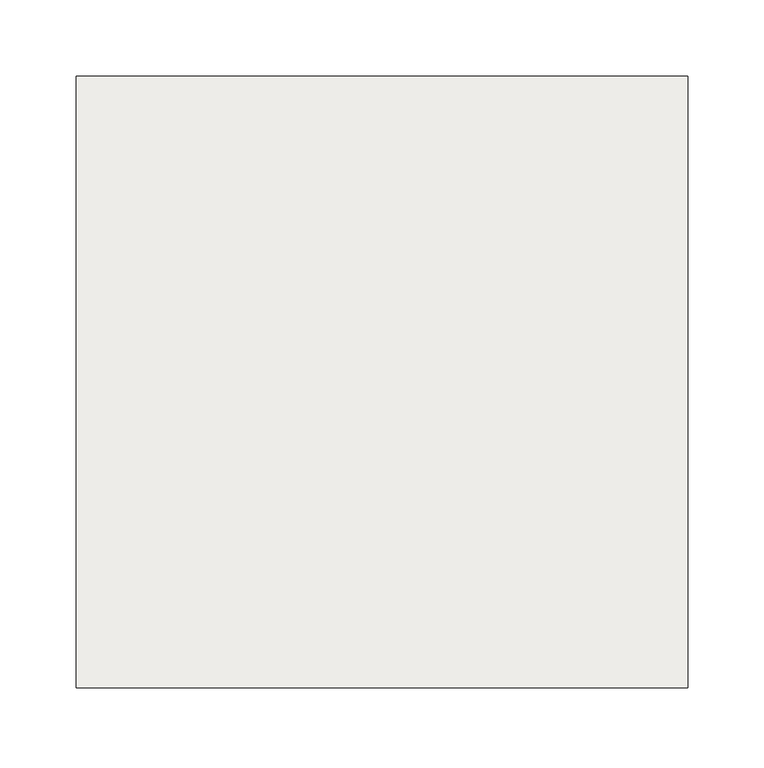
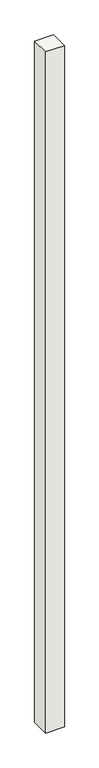
"""IFC4 building model written with IfcOpenShell, lengths in millimetres: slab geometry, NLRS_17_SFO_TLB_funderingspaal geheid beton prefab-AV-MMBPC_gen_rsf : heipaal beton prefab_gen__bxh 400x400."""

import ifcopenshell
import ifcopenshell.guid

model = None  # the IFC model being written
_history = None  # IfcOwnerHistory: only IFC2X3 demands one
_inside = {}  # id of a spatial element -> (the spatial element, [elements in it])
_under = {}  # id of a project, library or spatial element -> (it, [spatial elements below it])
_declared = {}  # id of a project -> (the project, [libraries it declares])
_typed = {}  # id of a type object -> (the type object, [elements of that type])
_made_of = {}  # id of a material, layer set ... -> (it, [elements and type objects made of it])


def new_model(schema):
    """Start an empty IFC model of exactly this schema.

    Asked for "IFC4X3", IfcOpenShell would pick the latest addendum, in which some entities
    have other attributes; the version numbers below select the first issue.
    IFC2X3 requires an IfcOwnerHistory on every rooted entity: one is made here for all.
    """
    global model, _history
    if schema == "IFC4X3":
        model = ifcopenshell.file(schema_version=(4, 3, 0, 0))
    else:
        model = ifcopenshell.file(schema=schema)
    _inside.clear()
    _under.clear()
    _declared.clear()
    _typed.clear()
    _made_of.clear()
    _history = None
    if model.schema == "IFC2X3":
        org = make("IfcOrganization", Name="unknown")
        user = make(
            "IfcPersonAndOrganization",
            ThePerson=make("IfcPerson", FamilyName="unknown"),
            TheOrganization=org,
        )
        app = make(
            "IfcApplication",
            ApplicationDeveloper=org,
            Version="unknown",
            ApplicationFullName="unknown",
            ApplicationIdentifier="unknown",
        )
        _history = make(
            "IfcOwnerHistory",
            OwningUser=user,
            OwningApplication=app,
            ChangeAction="ADDED",
            CreationDate=0,
        )
    return model


def make(cls, **values):
    """One entity of the class cls with the attributes given. An attribute that is None is left unset."""
    return model.create_entity(
        cls, **{name: value for name, value in values.items() if value is not None}
    )


def rooted(cls, **values):
    """An entity with a GlobalId (a new one), such as an element, a storey or a relation."""
    return make(cls, GlobalId=ifcopenshell.guid.new(), OwnerHistory=_history, **values)


def si_unit(unit_type, name, prefix=None):
    """IfcSIUnit, for example si_unit("LENGTHUNIT", "METRE", prefix="MILLI")."""
    return make("IfcSIUnit", UnitType=unit_type, Prefix=prefix, Name=name)


def assignment(units):
    """IfcUnitAssignment: the units of a project."""
    return None if units is None else make("IfcUnitAssignment", Units=units)


def point(xyz):
    """IfcCartesianPoint."""
    return None if xyz is None else make("IfcCartesianPoint", Coordinates=xyz)


def direction(xyz):
    """IfcDirection."""
    return None if xyz is None else make("IfcDirection", DirectionRatios=xyz)


def frame(location, z_axis=None, x_axis=None):
    """IfcAxis2Placement3D, a coordinate frame: its origin and axes. An axis left out is left unset."""
    return make(
        "IfcAxis2Placement3D",
        Location=point(location),
        Axis=direction(z_axis),
        RefDirection=direction(x_axis),
    )


def origin():
    """The frame at (0, 0, 0) with its axes left unset."""
    return frame((0.0, 0.0, 0.0))


def place(relative_to, where):
    """IfcLocalPlacement: puts the frame where relative to a parent placement (None: the world)."""
    return make(
        "IfcLocalPlacement", PlacementRelTo=relative_to, RelativePlacement=where
    )


def context(
    kind, dimensions, precision=None, world=None, true_north=None, identifier=None
):
    """IfcGeometricRepresentationContext, for example the 3D "Model" context."""
    return make(
        "IfcGeometricRepresentationContext",
        ContextIdentifier=identifier,
        ContextType=kind,
        CoordinateSpaceDimension=dimensions,
        Precision=precision,
        WorldCoordinateSystem=world,
        TrueNorth=true_north,
    )


def project(units=None, contexts=None):
    """IfcProject with its units and contexts."""
    return rooted(
        "IfcProject",
        Name="project",
        RepresentationContexts=contexts,
        UnitsInContext=assignment(units),
    )


def spatial(cls, under=None, at=None, **own):
    """A site, building, storey or space (cls), placed at a placement, below another one or the project."""
    s = rooted(cls, ObjectPlacement=at, **own)
    if under is not None:
        _under.setdefault(under.id(), (under, []))[1].append(s)
    return s


def polyline(points):
    """IfcPolyline through the points."""
    return make("IfcPolyline", Points=[point(p) for p in points])


def outline(outer, holes=None, kind="AREA"):
    """IfcArbitraryClosedProfileDef: a profile drawn as a closed curve; with holes, ...WithVoids."""
    if holes is None:
        return make("IfcArbitraryClosedProfileDef", ProfileType=kind, OuterCurve=outer)
    return make(
        "IfcArbitraryProfileDefWithVoids",
        ProfileType=kind,
        OuterCurve=outer,
        InnerCurves=holes,
    )


def extrude(swept, where, along, depth):
    """IfcExtrudedAreaSolid: the profile swept, set in the frame where, extruded along a direction by depth."""
    return make(
        "IfcExtrudedAreaSolid",
        SweptArea=swept,
        Position=where,
        ExtrudedDirection=direction(along),
        Depth=depth,
    )


def shape(context_of_items, identifier, shape_type, items):
    """IfcShapeRepresentation: the items that make up one representation, for example the "Body"."""
    return make(
        "IfcShapeRepresentation",
        ContextOfItems=context_of_items,
        RepresentationIdentifier=identifier,
        RepresentationType=shape_type,
        Items=items,
    )


def source(mapping_origin, context_of_items, identifier, shape_type, items):
    """IfcRepresentationMap: a shape defined once, which mapped items show again and again."""
    return make(
        "IfcRepresentationMap",
        MappingOrigin=mapping_origin,
        MappedRepresentation=shape(context_of_items, identifier, shape_type, items),
    )


def transform(
    local_origin,
    x_axis=None,
    y_axis=None,
    z_axis=None,
    scale=None,
    scale2=None,
    scale3=None,
    uniform=True,
):
    """IfcCartesianTransformationOperator3D, or its non-uniform kind. x_axis, y_axis, z_axis: its Axis1, 2, 3."""
    if uniform:
        return make(
            "IfcCartesianTransformationOperator3D",
            Axis1=direction(x_axis),
            Axis2=direction(y_axis),
            LocalOrigin=point(local_origin),
            Scale=scale,
            Axis3=direction(z_axis),
        )
    return make(
        "IfcCartesianTransformationOperator3DnonUniform",
        Axis1=direction(x_axis),
        Axis2=direction(y_axis),
        LocalOrigin=point(local_origin),
        Scale=scale,
        Axis3=direction(z_axis),
        Scale2=scale2,
        Scale3=scale3,
    )


def mapped(mapping_source, mapping_target):
    """IfcMappedItem: shows the shape of a source again, moved by a transform."""
    return make(
        "IfcMappedItem", MappingSource=mapping_source, MappingTarget=mapping_target
    )


def made_of(thing, what):
    """Note that an element or type object is made of a material, layer set ...; save() writes the relation."""
    if what is not None:
        _made_of.setdefault(what.id(), (what, []))[1].append(thing)
    return thing


def element(
    cls,
    number,
    at=None,
    inside=None,
    cuts=None,
    type_object=None,
    material=None,
    context=None,
    identifier="Body",
    shape_type=None,
    held_by="IfcProductDefinitionShape",
    body=None,
    shapes=None,
    **own,
):
    """One element of the class cls, such as IfcWall. Its Tag is "e" and its number.

    at: its placement. inside: the storey or other place that contains it. cuts: it is an
    opening in that element (IfcRelVoidsElement). A single representation is given by context,
    identifier, shape_type and body (its items); several are given by shapes. held_by: the class
    of the entity that holds the representations. save() writes the other relations.
    """
    e = rooted(cls, Tag="e%d" % number, ObjectPlacement=at, **own)
    if body is not None:
        shapes = [shape(context, identifier, shape_type, body)]
    if shapes is not None:
        e.Representation = make(held_by, Representations=shapes)
    if inside is not None:
        _inside.setdefault(inside.id(), (inside, []))[1].append(e)
    if cuts is not None:
        rooted(
            "IfcRelVoidsElement", RelatingBuildingElement=cuts, RelatedOpeningElement=e
        )
    if type_object is not None:
        _typed.setdefault(type_object.id(), (type_object, []))[1].append(e)
    return made_of(e, material)


def aggregate(whole, parts):
    """IfcRelAggregates: a whole, such as a stair, and the parts it consists of."""
    return rooted("IfcRelAggregates", RelatingObject=whole, RelatedObjects=parts)


def save(model, path):
    """Write the relations noted so far, then the file.

    IfcRelAggregates (storeys below a building ...), IfcRelContainedInSpatialStructure (elements
    in a storey), IfcRelDefinesByType, IfcRelAssociatesMaterial and IfcRelDeclares: one each for
    every whole, place, type object, material and project.
    """
    for whole, parts in _under.values():
        aggregate(whole, parts)
    for where, things in _inside.values():
        rooted(
            "IfcRelContainedInSpatialStructure",
            RelatedElements=things,
            RelatingStructure=where,
        )
    for kind, things in _typed.values():
        rooted("IfcRelDefinesByType", RelatedObjects=things, RelatingType=kind)
    for what, things in _made_of.values():
        rooted("IfcRelAssociatesMaterial", RelatedObjects=things, RelatingMaterial=what)
    for by, libraries in _declared.values():
        rooted("IfcRelDeclares", RelatingContext=by, RelatedDefinitions=libraries)
    model.write(path)


def slab_e3f33549(model_context):
    return source(origin(), model_context, "Body", "SweptSolid", [
        extrude(outline(polyline([(200.0, -200.0), (-200.0, -200.0), (-200.0, 200.0), (200.0, 200.0), (200.0, -200.0)])), frame((0.0, 0.0, -20000.0), z_axis=(0.0, 0.0, 1.0), x_axis=(1.0, 0.0, 0.0)), (0.0, 0.0, 1.0), 15320.0),
    ])


if __name__ == "__main__":
    model = new_model("IFC4")
    model_context = context("Model", 3, world=origin())
    ifc_project = project(units=[si_unit("LENGTHUNIT", "METRE", prefix="MILLI")], contexts=[model_context])
    site = spatial("IfcSite", under=ifc_project)
    building = spatial("IfcBuilding", under=site)
    placement = place(None, origin())
    slab_shape = slab_e3f33549(model_context)
    element("IfcSlab", 1, ObjectType="NLRS_17_SFO_TLB_funderingspaal geheid beton prefab-AV-MMBPC_gen_rsf : heipaal beton prefab_gen__bxh 400x400", at=placement, inside=building, context=model_context, shape_type="MappedRepresentation", body=[
        mapped(slab_shape, transform((0.0, 0.0, 0.0), x_axis=(1.0, 0.0, 0.0), y_axis=(0.0, 1.0, 0.0), z_axis=(0.0, 0.0, 1.0))),
    ])
    save(model, "model.ifc")

# Revit data of these elements
# Type "NLRS_17_SFO_TLB_funderingspaal geheid beton prefab-AV-MMBPC_gen_rsf : heipaal beton prefab_gen__bxh 400x400"
#   Export Type to IFC As = "IfcPile"
#   Type IfcGUID = "10$Kfo5uPCAOPJEOo5LE_W"
#   Type Comments = "prefab heipaal 400x400"
#   Model = " "
#   Manufacturer = " "
#   Description = "prefab heipaal 400x400"
#   Assembly Code = "17.21"
#   Width = 400 mm
#   Slanted Angle [instance default] = 0.00°
#   NLRS_S_draagvermogen_trek [instance default] = 0.00 kN
#   NLRS_S_draagvermogen_druk [instance default] = 0.00 kN
#   NLRS_C_lengte [instance default] = 1660 mm
#   NLRS_C_hoogte = 400 mm
#   NLRS_C_breedte = 400 mm
#   Height [instance default] = 1660 mm
#   Length [instance default] = 1660 mm
#   Angle [instance default] = 0.00°
#   Slanted [instance default] = 0
#   Structural Material = NLRS_f2_beton prefab_gen_rsf
#   Keynote = ""
# Element 1 (IfcSlab, "NLRS_17_SFO_TLB_funderingspaal geheid beton prefab-AV-MMBPC_gen_rsf : heipaal beton prefab_gen__bxh 400x400")
#   NLRS_C_lengte = 15320 mm
#   Height = 15320 mm
#   Length = 15320 mm
#   Materials on its faces: "NLRS_f2_beton prefab_gen_rsf"
# Materials
#   "NLRS_f2_beton prefab_gen_rsf": class "F - Niet gebakken kunststeen", colour RGB 129 133 118, transparency 0, Keynote = "f2", Manufacturer = "Revit Standards Foundation", URL = "www.revitstandards.org", Description = "beton prefab", Cost = 0
